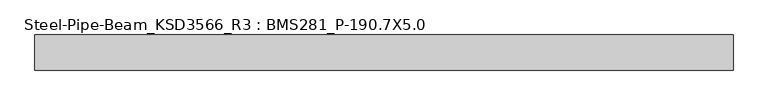
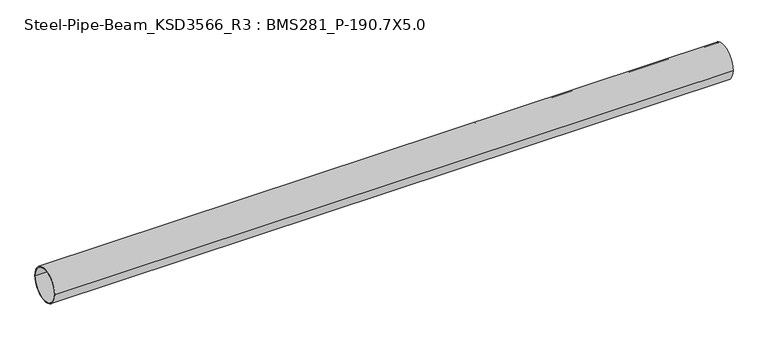
"""IFC4 building model written with IfcOpenShell, lengths in millimetres: member geometry, Steel-Pipe-Beam_KSD3566_R3 : BMS281_P-190.7X5.0."""

from ifc_helpers import new_model, si_unit, point, frame, origin, origin_2d, place, context, project, spatial, circle_curve, trimmed, segment, composite_curve, outline, extrude, source, transform, mapped, element, save


def steel_pipe_beam_ksd3566_r3_bms281_p_190_7x5_0_c82f9055(model_context):
    return source(origin(), model_context, "Body", "SweptSolid", [
        extrude(outline(composite_curve([segment(trimmed(circle_curve(origin_2d(), 95.35), [point((-95.35, 0.0))], [point((95.35, 0.0))], False, "CARTESIAN"), True, "CONTINUOUS"), segment(trimmed(circle_curve(origin_2d(), 95.35), [point((95.35, 0.0))], [point((-95.35, 0.0))], False, "CARTESIAN"), True, "CONTINUOUS")], self_intersect=False), holes=[composite_curve([segment(trimmed(circle_curve(origin_2d(), 90.35), [point((90.35, 0.0))], [point((-90.35, 0.0))], True, "CARTESIAN"), True, "CONTINUOUS"), segment(trimmed(circle_curve(origin_2d(), 90.35), [point((-90.35, 0.0))], [point((90.35, 0.0))], True, "CARTESIAN"), True, "CONTINUOUS")], self_intersect=False)]), frame((-1887.8910773, 0.0, 0.0), z_axis=(1.0, 0.0, 0.0), x_axis=(0.0, 1.0, 0.0)), (0.0, 0.0, 1.0), 3789.2307634),
    ])


if __name__ == "__main__":
    model = new_model("IFC4")
    model_context = context("Model", 3, world=origin())
    ifc_project = project(units=[si_unit("LENGTHUNIT", "METRE", prefix="MILLI")], contexts=[model_context])
    site = spatial("IfcSite", under=ifc_project)
    building = spatial("IfcBuilding", under=site)
    placement = place(None, origin())
    steel_pipe_beam_ksd3566_r3_bms281_p_190_7x5_0_shape = steel_pipe_beam_ksd3566_r3_bms281_p_190_7x5_0_c82f9055(model_context)
    element("IfcMember", 1, ObjectType="Steel-Pipe-Beam_KSD3566_R3 : BMS281_P-190.7X5.0", at=placement, inside=building, context=model_context, shape_type="MappedRepresentation", body=[
        mapped(steel_pipe_beam_ksd3566_r3_bms281_p_190_7x5_0_shape, transform((0.0, 0.0, 0.0), x_axis=(1.0, 0.0, 0.0), y_axis=(0.0, 1.0, 0.0), z_axis=(0.0, 0.0, 1.0))),
    ])
    save(model, "model.ifc")

# Revit data of these elements
# Type "Steel-Pipe-Beam_KSD3566_R3 : BMS281_P-190.7X5.0"
#   Keynote = "P-190.7X5.0"
#   SteelWeight = "Light"
#   t = 0.0050 m
#   Surface Area = 0.599102 m²/m
#   Section Area = 29.1697 cm²
#   Mass per Unit Length = 22.8982 kg/m
#   Length [instance default] = 1.5000 m
#   D = 0.1907 m
#   hec_material4 [instance default] = none
#   hec_material3 [instance default] = none
#   hec_material2 [instance default] = none
#   hec_material1 [instance default] = none
#   Structural Material [instance default] = Steel, 45-345
#   Assembly Code = ""
# Element 1 (IfcMember, "Steel-Pipe-Beam_KSD3566_R3 : BMS281_P-190.7X5.0")
#   Structural Material = none
# Materials
#   "Steel, 45-345": class "Metal", colour RGB 189 187 185, transparency 0, Description = "Steel 345 MPa", Cost = 0
